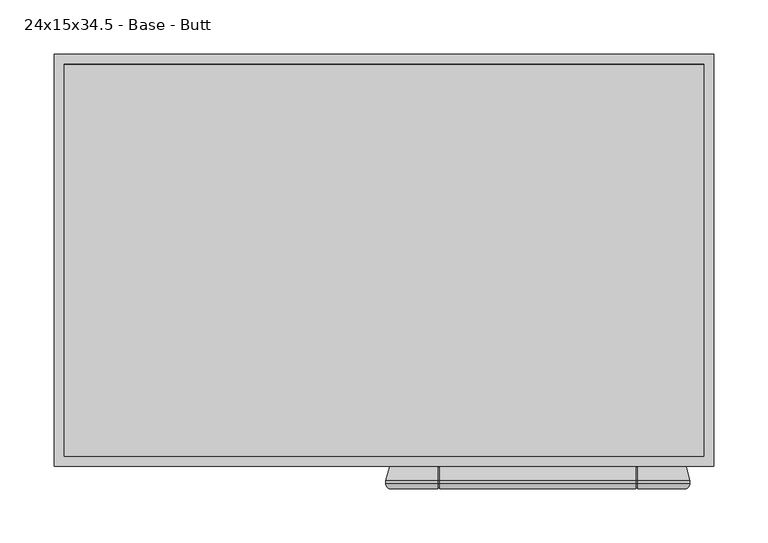
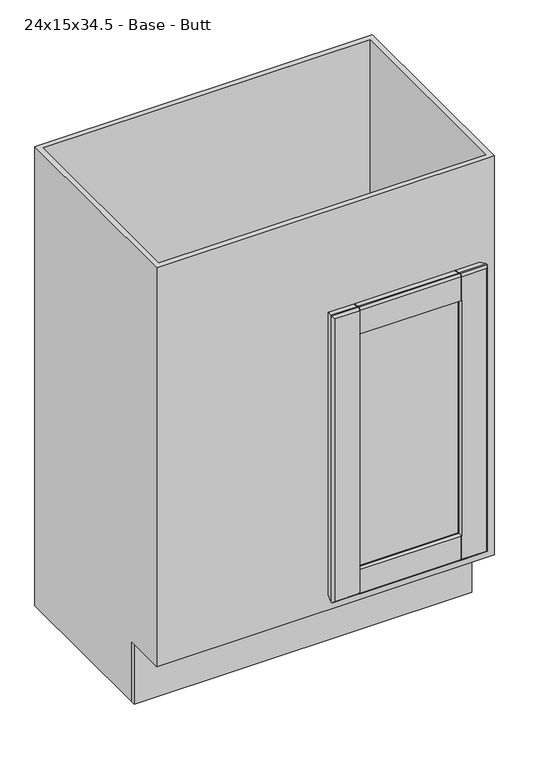
"""IFC4 building model written with IfcOpenShell, lengths in millimetres: furniture geometry, Cabinet-Base-Merillat-Double_Door-Marlin : 24x15x34.5 - Base - Butt."""

from ifc_helpers import new_model, si_unit, frame, origin, origin_with_axes, place, context, project, spatial, polyline, circle_curve, ellipse_curve, outline, extrude, faceted_brep, source, transform, mapped, element, save
from ifc_brep_helpers import plane_surface, cylinder_surface, advanced_brep


def furniture_24x15x34_5_base_butt_ddcd1996(model_context):
    return source(origin(), model_context, "Body", "SolidModel", [
        advanced_brep(
        [(301.3127049, -625.4496, 685.8), (298.2162124, -629.92, 682.7035075), (298.2162124, -629.92, 142.7964925), (301.3127049, -625.4496, 139.7), (301.3127049, -622.681, 139.7), (301.3127049, -622.681, 685.8), (297.8075049, -609.6, 143.2052), (297.8075049, -609.6, 682.2948), (253.1115422, -609.6, 637.5988372), (253.1115422, -609.6, 187.9011628), (252.7414105, -610.39375, 188.2712945), (250.6602514, -614.85681, 190.3524535), (250.6602514, -614.85681, 635.1475465), (252.7414105, -610.39375, 637.2287055), (252.0600209, -617.0969093, 188.952684), (252.0600209, -617.0969093, 636.547316), (266.3877049, -617.347, 174.625), (266.3877049, -617.347, 650.875), (266.3877049, -622.173, 174.625), (266.3877049, -622.173, 650.875), (252.0600209, -622.4230907, 188.952684), (252.0600209, -622.4230907, 636.547316), (250.6602514, -624.66319, 190.3524535), (250.6602514, -624.66319, 635.1475465), (252.7414105, -629.12625, 188.2712945), (253.1086747, -629.9138508, 187.9040302), (253.1115422, -629.92, 637.5988372), (252.7414105, -629.12625, 637.2287055), (253.1086747, -629.92, 142.7964925), (253.1086747, -625.4496, 139.7), (23.4216974, -629.92, 142.7964925), (20.3252049, -625.4496, 139.7), (68.4894236, -625.4496, 139.7), (68.4894236, -629.92, 142.7964925), (251.5211747, -625.4496, 139.7), (251.5211747, -629.92, 142.7964925), (70.0769236, -629.92, 142.7964925), (70.0769236, -625.4496, 139.7), (253.1086747, -622.681, 139.7), (20.3252049, -622.681, 139.7), (68.4894236, -622.681, 139.7), (251.5211747, -622.681, 139.7), (70.0769236, -622.681, 139.7), (253.1086747, -609.6, 143.2052), (23.8304049, -609.6, 143.2052), (68.4894236, -609.6, 143.2052), (251.5211747, -609.6, 143.2052), (70.0769236, -609.6, 143.2052), (70.9776584, -614.85681, 190.3524535), (251.5211747, -610.39375, 188.2712945), (251.5211747, -609.6, 187.9011628), (70.0769236, -609.6, 187.9011628), (70.0769236, -610.39375, 188.2712945), (68.8964994, -610.39375, 188.2712945), (69.577889, -617.0969093, 188.952684), (55.2502049, -617.347, 174.625), (55.2502049, -622.173, 174.625), (69.577889, -622.4230907, 188.952684), (70.9776584, -624.66319, 190.3524535), (68.8964994, -629.12625, 188.2712945), (70.0769236, -629.12625, 188.2712945), (70.0769236, -629.92, 187.9011628), (251.5211747, -629.92, 187.9011628), (251.5211747, -629.12625, 188.2712945), (23.4216974, -629.92, 682.7035075), (20.3252049, -625.4496, 685.8), (20.3252049, -622.681, 685.8), (23.8304049, -609.6, 682.2948), (68.5263677, -609.6, 187.9011628), (68.5263677, -609.6, 637.5988372), (68.8964994, -610.39375, 637.2287055), (70.9776584, -614.85681, 635.1475465), (69.577889, -617.0969093, 636.547316), (55.2502049, -617.347, 650.875), (55.2502049, -622.173, 650.875), (69.577889, -622.4230907, 636.547316), (70.9776584, -624.66319, 635.1475465), (68.8964994, -629.12625, 637.2287055), (68.5263677, -629.92, 637.5988372), (68.5263677, -629.92, 187.9011628), (68.4894236, -629.92, 682.7035075), (68.4894236, -625.4496, 685.8), (253.1086747, -625.4496, 685.8), (253.1086747, -629.92, 682.7035075), (70.0769236, -625.4496, 685.8), (70.0769236, -629.92, 682.7035075), (251.5211747, -629.92, 682.7035075), (251.5211747, -625.4496, 685.8), (68.4894236, -622.681, 685.8), (253.1086747, -622.681, 685.8), (70.0769236, -622.681, 685.8), (251.5211747, -622.681, 685.8), (68.4894236, -609.6, 682.2948), (253.1086747, -609.6, 682.2948), (70.0769236, -609.6, 682.2948), (251.5211747, -609.6, 682.2948), (70.0769236, -609.6, 637.5988372), (251.5211747, -609.6, 637.5988372), (70.0769236, -610.39375, 637.2287055), (251.5211747, -610.39375, 637.2287055), (251.5211747, -629.12625, 637.2287055), (251.5211747, -629.92, 637.5988372), (70.0769236, -629.92, 637.5988372), (70.0769236, -629.12625, 637.2287055), (70.0769236, -610.39375, 681.6857412), (70.0769236, -622.7855037, 685.00625), (70.0769236, -625.4496, 685.00625), (70.0769236, -629.12625, 682.5526052), (68.4894236, -629.12625, 637.2287055), (68.4894236, -629.12625, 682.5526052), (68.4894236, -625.4496, 685.00625), (68.4894236, -622.7855037, 685.00625), (68.4894236, -610.39375, 681.6857412), (68.4894236, -610.39375, 637.2287055), (253.1086747, -610.39375, 637.2287055), (253.1086747, -610.39375, 681.6857412), (253.1086747, -622.7855037, 685.00625), (253.1086747, -625.4496, 685.00625), (253.1086747, -629.12625, 682.5526052), (253.1086747, -629.12625, 637.2287055), (251.5211747, -629.12625, 682.5526052), (251.5211747, -625.4496, 685.00625), (251.5211747, -622.7855037, 685.00625), (251.5211747, -610.39375, 681.6857412), (253.1086747, -629.12625, 188.2712945), (253.1086747, -629.12625, 142.9473948), (253.1086747, -625.4496, 140.49375), (253.1086747, -622.7855037, 140.49375), (253.1086747, -610.39375, 143.8142588), (253.1086747, -610.39375, 188.2712945), (251.5211747, -610.39375, 143.8142588), (251.5211747, -622.7855037, 140.49375), (251.5211747, -625.4496, 140.49375), (251.5211747, -629.12625, 142.9473948), (70.0769236, -629.12625, 142.9473948), (70.0769236, -625.4496, 140.49375), (70.0769236, -622.7855037, 140.49375), (70.0769236, -610.39375, 143.8142588), (68.4894236, -629.12625, 188.2712945), (68.4894236, -610.39375, 188.2712945), (68.4894236, -610.39375, 143.8142588), (68.4894236, -622.7855037, 140.49375), (68.4894236, -625.4496, 140.49375), (68.4894236, -629.12625, 142.9473948)],
        [
            (0, 1, ellipse_curve(frame((296.5375049, -625.4496, 681.0248), z_axis=(0.7071067811865475, 0.0, -0.7071067811865475), x_axis=(0.7071067811865474, 0.0, 0.7071067811865476)), 6.7531526, 4.7752)),
            (1, 2),
            (2, 3, ellipse_curve(frame((296.5375049, -625.4496, 144.4752), z_axis=(0.7071067811865475, 0.0, 0.7071067811865475), x_axis=(-0.7071067811865474, 0.0, 0.7071067811865476)), 6.7531526, 4.7752)),
            (3, 0),
            (3, 4),
            (4, 5),
            (5, 0),
            (4, 6),
            (6, 7),
            (7, 5),
            (8, 9),
            (9, 10),
            (10, 11),
            (11, 12),
            (12, 13),
            (13, 8),
            (11, 14, ellipse_curve(frame((252.0875049, -615.5223492, 188.9252), z_axis=(0.7071067811865475, 0.0, 0.7071067811865475), x_axis=(-0.7071067811865474, 0.0, 0.7071067811865476)), 2.2271035, 1.5748)),
            (14, 15),
            (15, 12, ellipse_curve(frame((252.0875049, -615.5223492, 636.5748), z_axis=(0.7071067811865475, 0.0, -0.7071067811865475), x_axis=(0.7071067811865474, 0.0, 0.7071067811865476)), 2.2271035, 1.5748)),
            (14, 16),
            (16, 17),
            (17, 15),
            (16, 18),
            (18, 19),
            (19, 17),
            (18, 20),
            (20, 21),
            (21, 19),
            (20, 22, ellipse_curve(frame((252.0875049, -623.9976508, 188.9252), z_axis=(0.7071067811865475, 0.0, 0.7071067811865475), x_axis=(-0.7071067811865474, 0.0, 0.7071067811865476)), 2.2271035, 1.5748)),
            (22, 23),
            (23, 21, ellipse_curve(frame((252.0875049, -623.9976508, 636.5748), z_axis=(0.7071067811865475, 0.0, -0.7071067811865475), x_axis=(0.7071067811865474, 0.0, 0.7071067811865476)), 2.2271035, 1.5748)),
            (22, 24),
            (24, 25),
            (25, 26),
            (26, 27),
            (27, 23),
            (2, 28),
            (28, 29, circle_curve(frame((253.1086747, -625.4496, 144.4752), z_axis=(1.0, 0.0, 0.0), x_axis=(0.0, 1.0, 0.0)), 4.7752)),
            (29, 3),
            (30, 31, ellipse_curve(frame((25.1004049, -625.4496, 144.4752), z_axis=(0.7071067811865475, 0.0, -0.7071067811865475), x_axis=(0.7071067811865476, 0.0, 0.7071067811865474)), 6.7531526, 4.7752)),
            (31, 32),
            (32, 33, circle_curve(frame((68.4894236, -625.4496, 144.4752), z_axis=(-1.0, 0.0, 0.0), x_axis=(0.0, 1.0, 0.0)), 4.7752)),
            (33, 30),
            (34, 35, circle_curve(frame((251.5211747, -625.4496, 144.4752), z_axis=(-1.0, 0.0, 0.0), x_axis=(0.0, 1.0, 0.0)), 4.7752)),
            (35, 36),
            (36, 37, circle_curve(frame((70.0769236, -625.4496, 144.4752), z_axis=(1.0, 0.0, 0.0), x_axis=(0.0, 1.0, 0.0)), 4.7752)),
            (37, 34),
            (29, 38),
            (38, 4),
            (31, 39),
            (39, 40),
            (40, 32),
            (41, 34),
            (37, 42),
            (42, 41),
            (38, 43),
            (43, 6),
            (39, 44),
            (44, 45),
            (45, 40),
            (46, 41),
            (42, 47),
            (47, 46),
            (48, 11),
            (10, 49),
            (49, 50),
            (50, 51),
            (51, 52),
            (52, 53),
            (53, 48),
            (48, 54, ellipse_curve(frame((69.5504049, -615.5223492, 188.9252), z_axis=(0.7071067811865475, 0.0, -0.7071067811865475), x_axis=(0.7071067811865476, 0.0, 0.7071067811865474)), 2.2271035, 1.5748)),
            (54, 14),
            (54, 55),
            (55, 16),
            (55, 56),
            (56, 18),
            (56, 57),
            (57, 20),
            (57, 58, ellipse_curve(frame((69.5504049, -623.9976508, 188.9252), z_axis=(0.7071067811865475, 0.0, -0.7071067811865475), x_axis=(0.7071067811865476, 0.0, 0.7071067811865474)), 2.2271035, 1.5748)),
            (58, 22),
            (58, 59),
            (59, 60),
            (60, 61),
            (61, 62),
            (62, 63),
            (63, 24),
            (30, 64),
            (64, 65, ellipse_curve(frame((25.1004049, -625.4496, 681.0248), z_axis=(-0.7071067811865475, 0.0, -0.7071067811865475), x_axis=(0.7071067811865474, 0.0, -0.7071067811865476)), 6.7531526, 4.7752)),
            (65, 31),
            (65, 66),
            (66, 39),
            (66, 67),
            (67, 44),
            (68, 69),
            (69, 70),
            (70, 71),
            (71, 48),
            (53, 68),
            (71, 72, ellipse_curve(frame((69.5504049, -615.5223492, 636.5748), z_axis=(-0.7071067811865475, 0.0, -0.7071067811865475), x_axis=(0.7071067811865474, 0.0, -0.7071067811865476)), 2.2271035, 1.5748)),
            (72, 54),
            (72, 73),
            (73, 55),
            (73, 74),
            (74, 56),
            (74, 75),
            (75, 57),
            (75, 76, ellipse_curve(frame((69.5504049, -623.9976508, 636.5748), z_axis=(-0.7071067811865475, 0.0, -0.7071067811865475), x_axis=(0.7071067811865474, 0.0, -0.7071067811865476)), 2.2271035, 1.5748)),
            (76, 58),
            (76, 77),
            (77, 78),
            (78, 79),
            (79, 59),
            (64, 80),
            (80, 81, circle_curve(frame((68.4894236, -625.4496, 681.0248), z_axis=(-1.0, 0.0, 0.0), x_axis=(0.0, 1.0, 0.0)), 4.7752)),
            (81, 65),
            (0, 82),
            (82, 83, circle_curve(frame((253.1086747, -625.4496, 681.0248), z_axis=(1.0, 0.0, 0.0), x_axis=(0.0, 1.0, 0.0)), 4.7752)),
            (83, 1),
            (84, 85, circle_curve(frame((70.0769236, -625.4496, 681.0248), z_axis=(1.0, 0.0, 0.0), x_axis=(0.0, 1.0, 0.0)), 4.7752)),
            (85, 86),
            (86, 87, circle_curve(frame((251.5211747, -625.4496, 681.0248), z_axis=(-1.0, 0.0, 0.0), x_axis=(0.0, 1.0, 0.0)), 4.7752)),
            (87, 84),
            (81, 88),
            (88, 66),
            (5, 89),
            (89, 82),
            (90, 84),
            (87, 91),
            (91, 90),
            (88, 92),
            (92, 67),
            (7, 93),
            (93, 89),
            (94, 90),
            (91, 95),
            (95, 94),
            (43, 9),
            (8, 93),
            (92, 69),
            (68, 45),
            (96, 94),
            (95, 97),
            (97, 96),
            (50, 46),
            (47, 51),
            (12, 71),
            (70, 98),
            (98, 96),
            (97, 99),
            (99, 13),
            (15, 72),
            (17, 73),
            (19, 74),
            (21, 75),
            (23, 76),
            (27, 100),
            (100, 101),
            (101, 102),
            (102, 103),
            (103, 77),
            (83, 26),
            (25, 28),
            (33, 79),
            (78, 80),
            (85, 102),
            (101, 86),
            (35, 62),
            (61, 36),
            (98, 104),
            (104, 105),
            (105, 106),
            (106, 107, circle_curve(frame((70.0769236, -625.4496, 681.0248), z_axis=(1.0, 0.0, 0.0), x_axis=(0.0, 0.0, 1.0)), 3.98145)),
            (107, 103),
            (78, 108),
            (108, 109),
            (109, 110, circle_curve(frame((68.4894236, -625.4496, 681.0248), z_axis=(-1.0, 0.0, 0.0), x_axis=(0.0, 0.0, 1.0)), 3.98145)),
            (110, 111),
            (111, 112),
            (112, 113),
            (113, 69),
            (77, 108),
            (107, 109),
            (106, 110),
            (105, 111),
            (104, 112),
            (70, 113),
            (8, 114),
            (114, 115),
            (115, 116),
            (116, 117),
            (117, 118, circle_curve(frame((253.1086747, -625.4496, 681.0248), z_axis=(1.0, 0.0, 0.0), x_axis=(0.0, 0.0, 1.0)), 3.98145)),
            (118, 119),
            (119, 26),
            (100, 120),
            (120, 121, circle_curve(frame((251.5211747, -625.4496, 681.0248), z_axis=(-1.0, 0.0, 0.0), x_axis=(0.0, 0.0, 1.0)), 3.98145)),
            (121, 122),
            (122, 123),
            (123, 99),
            (119, 27),
            (118, 120),
            (117, 121),
            (116, 122),
            (115, 123),
            (114, 13),
            (25, 124),
            (124, 125),
            (125, 126, circle_curve(frame((253.1086747, -625.4496, 144.4752), z_axis=(1.0, 0.0, 0.0), x_axis=(0.0, 0.0, 1.0)), 3.98145)),
            (126, 127),
            (127, 128),
            (128, 129),
            (129, 9),
            (49, 130),
            (130, 131),
            (131, 132),
            (132, 133, circle_curve(frame((251.5211747, -625.4496, 144.4752), z_axis=(-1.0, 0.0, 0.0), x_axis=(0.0, 0.0, 1.0)), 3.98145)),
            (133, 63),
            (129, 10),
            (128, 130),
            (127, 131),
            (126, 132),
            (125, 133),
            (124, 24),
            (60, 134),
            (134, 135, circle_curve(frame((70.0769236, -625.4496, 144.4752), z_axis=(1.0, 0.0, 0.0), x_axis=(0.0, 0.0, 1.0)), 3.98145)),
            (135, 136),
            (136, 137),
            (137, 52),
            (138, 79),
            (68, 139),
            (139, 140),
            (140, 141),
            (141, 142),
            (142, 143, circle_curve(frame((68.4894236, -625.4496, 144.4752), z_axis=(-1.0, 0.0, 0.0), x_axis=(0.0, 0.0, 1.0)), 3.98145)),
            (143, 138),
            (138, 59),
            (53, 139),
            (137, 140),
            (136, 141),
            (135, 142),
            (134, 143),
        ],
        [
            cylinder_surface(frame((296.5375049, -625.4496, 685.8), z_axis=(0.0, 0.0, 1.0), x_axis=(0.0, 1.0, 0.0)), 4.7752),
            plane_surface(frame((301.3127049, -625.4496, 685.8), z_axis=(1.0, 0.0, 0.0), x_axis=(0.0, 0.0, -1.0))),
            plane_surface(frame((301.3127049, -622.681, 685.8), z_axis=(0.9659229350723619, 0.25882983502910506, 0.0), x_axis=(0.0, 0.0, -1.0))),
            plane_surface(frame((253.1115422, -609.6, 637.5988372), z_axis=(-0.9063077870366099, 0.4226182617407856, 0.0), x_axis=(0.0, 0.0, -1.0))),
            cylinder_surface(frame((252.0875049, -615.5223492, 685.8), z_axis=(0.0, 0.0, 1.0000000000000002), x_axis=(-0.01745240643729364, -0.9998476951563912, 0.0)), 1.5748),
            plane_surface(frame((252.0600209, -617.0969093, 636.547316), z_axis=(-0.017452406437322144, -0.9998476951563906, 0.0), x_axis=(0.0, 0.0, -1.0))),
            plane_surface(frame((266.3877049, -617.347, 650.875), z_axis=(-1.0, 0.0, 0.0), x_axis=(0.0, 0.0, -1.0))),
            plane_surface(frame((266.3877049, -622.173, 650.875), z_axis=(-0.01745240643727848, 0.9998476951563914, 0.0), x_axis=(0.0, 0.0, -1.0))),
            cylinder_surface(frame((252.0875049, -623.9976508, 685.8), z_axis=(0.0, 0.0, 1.0000000000000002), x_axis=(-0.9063077870367326, -0.42261826174052236, 0.0)), 1.5748),
            plane_surface(frame((250.6602514, -624.66319, 635.1475465), z_axis=(-0.9063077870366333, -0.4226182617407352, 0.0), x_axis=(0.0, 0.0, -1.0))),
            cylinder_surface(frame((301.3127049, -625.4496, 144.4752), z_axis=(1.0, 0.0, 0.0), x_axis=(0.0, 1.0, 0.0)), 4.7752),
            plane_surface(frame((301.3127049, -625.4496, 139.7), z_axis=(0.0, 0.0, -1.0), x_axis=(-1.0, 0.0, 0.0))),
            plane_surface(frame((301.3127049, -622.681, 139.7), z_axis=(0.0, 0.25882983502910506, -0.9659229350723619), x_axis=(-1.0, 0.0, 0.0))),
            plane_surface(frame((253.1115422, -609.6, 187.9011628), z_axis=(0.0, 0.4226182617407856, 0.9063077870366099), x_axis=(-1.0, 0.0, 0.0))),
            cylinder_surface(frame((301.3127049, -615.5223492, 188.9252), z_axis=(1.0000000000000002, 0.0, 0.0), x_axis=(0.0, -0.9998476951563912, 0.01745240643729364)), 1.5748),
            plane_surface(frame((252.0600209, -617.0969093, 188.952684), z_axis=(0.0, -0.9998476951563906, 0.017452406437322144), x_axis=(-1.0, 0.0, 0.0))),
            plane_surface(frame((266.3877049, -617.347, 174.625), z_axis=(0.0, 0.0, 1.0), x_axis=(-1.0, 0.0, 0.0))),
            plane_surface(frame((266.3877049, -622.173, 174.625), z_axis=(0.0, 0.9998476951563914, 0.01745240643727848), x_axis=(-1.0, 0.0, 0.0))),
            cylinder_surface(frame((301.3127049, -623.9976508, 188.9252), z_axis=(1.0000000000000002, 0.0, 0.0), x_axis=(0.0, -0.42261826174052236, 0.9063077870367326)), 1.5748),
            plane_surface(frame((250.6602514, -624.66319, 190.3524535), z_axis=(0.0, -0.4226182617407352, 0.9063077870366333), x_axis=(-1.0, 0.0, 0.0))),
            cylinder_surface(frame((25.1004049, -625.4496, 139.7), z_axis=(0.0, 0.0, -1.0), x_axis=(0.0, 1.0, 0.0)), 4.7752),
            plane_surface(frame((20.3252049, -625.4496, 139.7), z_axis=(-1.0, 0.0, 0.0), x_axis=(0.0, 0.0, 1.0))),
            plane_surface(frame((20.3252049, -622.681, 139.7), z_axis=(-0.9659229350723619, 0.25882983502910506, 0.0), x_axis=(0.0, 0.0, 1.0))),
            plane_surface(frame((68.5263677, -609.6, 187.9011628), z_axis=(0.9063077870366099, 0.4226182617407856, 0.0), x_axis=(0.0, 0.0, 1.0))),
            cylinder_surface(frame((69.5504049, -615.5223492, 139.7), z_axis=(0.0, 0.0, -1.0000000000000002), x_axis=(0.01745240643729364, -0.9998476951563912, 0.0)), 1.5748),
            plane_surface(frame((69.577889, -617.0969093, 188.952684), z_axis=(0.017452406437322144, -0.9998476951563906, 0.0), x_axis=(0.0, 0.0, 1.0))),
            plane_surface(frame((55.2502049, -617.347, 174.625), z_axis=(1.0, 0.0, 0.0), x_axis=(0.0, 0.0, 1.0))),
            plane_surface(frame((55.2502049, -622.173, 174.625), z_axis=(0.01745240643727848, 0.9998476951563914, 0.0), x_axis=(0.0, 0.0, 1.0))),
            cylinder_surface(frame((69.5504049, -623.9976508, 139.7), z_axis=(0.0, 0.0, -1.0000000000000002), x_axis=(0.9063077870367326, -0.42261826174052236, 0.0)), 1.5748),
            plane_surface(frame((70.9776584, -624.66319, 190.3524535), z_axis=(0.9063077870366333, -0.4226182617407352, 0.0), x_axis=(0.0, 0.0, 1.0))),
            cylinder_surface(frame((20.3252049, -625.4496, 681.0248), z_axis=(-1.0, 0.0, 0.0), x_axis=(0.0, 1.0, 0.0)), 4.7752),
            plane_surface(frame((20.3252049, -625.4496, 685.8), z_axis=(0.0, 0.0, 1.0), x_axis=(1.0, 0.0, 0.0))),
            plane_surface(frame((20.3252049, -622.681, 685.8), z_axis=(0.0, 0.25882983502910506, 0.9659229350723619), x_axis=(1.0, 0.0, 0.0))),
            plane_surface(frame((23.8304049, -609.6, 682.2948), z_axis=(0.0, 1.0, 0.0), x_axis=(1.0, 0.0, 0.0))),
            plane_surface(frame((68.5263677, -609.6, 637.5988372), z_axis=(0.0, 0.4226182617407856, -0.9063077870366099), x_axis=(1.0, 0.0, 0.0))),
            cylinder_surface(frame((20.3252049, -615.5223492, 636.5748), z_axis=(-1.0000000000000002, 0.0, 0.0), x_axis=(0.0, -0.9998476951563912, -0.01745240643729364)), 1.5748),
            plane_surface(frame((69.577889, -617.0969093, 636.547316), z_axis=(0.0, -0.9998476951563906, -0.017452406437322144), x_axis=(1.0, 0.0, 0.0))),
            plane_surface(frame((55.2502049, -617.347, 650.875), z_axis=(0.0, 0.0, -1.0), x_axis=(1.0, 0.0, 0.0))),
            plane_surface(frame((55.2502049, -622.173, 650.875), z_axis=(0.0, 0.9998476951563914, -0.01745240643727848), x_axis=(1.0, 0.0, 0.0))),
            cylinder_surface(frame((20.3252049, -623.9976508, 636.5748), z_axis=(-1.0000000000000002, 0.0, 0.0), x_axis=(0.0, -0.42261826174052236, -0.9063077870367326)), 1.5748),
            plane_surface(frame((70.9776584, -624.66319, 635.1475465), z_axis=(0.0, -0.4226182617407352, -0.9063077870366333), x_axis=(1.0, 0.0, 0.0))),
            plane_surface(frame((68.5263677, -629.92, 637.5988372), z_axis=(0.0, -1.0, 0.0), x_axis=(1.0, 0.0, 0.0))),
            plane_surface(frame((70.0769236, -629.92, 637.5988372), z_axis=(-1.0, 0.0, 0.0), x_axis=(0.0, 0.906307787036771, -0.4226182617404399))),
            plane_surface(frame((68.4894236, -629.92, 637.5988372), z_axis=(1.0, 0.0, 0.0), x_axis=(0.0, -0.906307787036771, 0.4226182617404399))),
            plane_surface(frame((70.0769236, -629.92, 637.5988372), z_axis=(0.0, 0.4226182617404399, 0.906307787036771), x_axis=(-1.0, 0.0, 0.0))),
            plane_surface(frame((70.0769236, -629.12625, 637.2287055), z_axis=(0.0, -1.0, 0.0), x_axis=(-1.0, 0.0, 0.0))),
            cylinder_surface(frame((68.4894236, -625.4496, 681.0248), z_axis=(-1.0, 0.0, 0.0), x_axis=(0.0, 0.0, 1.0)), 3.98145),
            plane_surface(frame((70.0769236, -625.4496, 685.00625), z_axis=(0.0, 0.0, 1.0), x_axis=(-1.0, 0.0, 0.0))),
            plane_surface(frame((70.0769236, -622.7855037, 685.00625), z_axis=(0.0, 0.25882983502913415, 0.9659229350723542), x_axis=(-1.0, 0.0, 0.0))),
            plane_surface(frame((70.0769236, -610.39375, 681.6857412), z_axis=(0.0, 1.0, 0.0), x_axis=(-1.0, 0.0, 0.0))),
            plane_surface(frame((70.0769236, -610.39375, 637.2287055), z_axis=(0.0, -0.4226182617405111, 0.9063077870367379), x_axis=(-1.0, 0.0, 0.0))),
            plane_surface(frame((253.1086747, -629.92, 637.5988372), z_axis=(-1.0, 0.0, 0.0), x_axis=(0.0, 0.9063077870367783, -0.42261826174042444))),
            plane_surface(frame((251.5211747, -629.92, 637.5988372), z_axis=(1.0, 0.0, 0.0), x_axis=(0.0, -0.9063077870367783, 0.42261826174042444))),
            plane_surface(frame((253.1086747, -629.92, 637.5988372), z_axis=(0.0, 0.42261826174042444, 0.9063077870367783), x_axis=(-1.0, 0.0, 0.0))),
            plane_surface(frame((253.1086747, -629.12625, 637.2287055), z_axis=(0.0, -1.0, 0.0), x_axis=(-1.0, 0.0, 0.0))),
            cylinder_surface(frame((251.5211747, -625.4496, 681.0248), z_axis=(-1.0, 0.0, 0.0), x_axis=(0.0, 0.0, 1.0)), 3.98145),
            plane_surface(frame((253.1086747, -625.4496, 685.00625), z_axis=(0.0, 0.0, 1.0), x_axis=(-1.0, 0.0, 0.0))),
            plane_surface(frame((253.1086747, -622.7855037, 685.00625), z_axis=(0.0, 0.25882983502911566, 0.965922935072359), x_axis=(-1.0, 0.0, 0.0))),
            plane_surface(frame((253.1086747, -610.39375, 681.6857412), z_axis=(0.0, 1.0, 0.0), x_axis=(-1.0, 0.0, 0.0))),
            plane_surface(frame((253.1086747, -610.39375, 637.2287055), z_axis=(0.0, -0.42261826174056427, 0.9063077870367131), x_axis=(-1.0, 0.0, 0.0))),
            plane_surface(frame((253.1086747, -625.4496, 149.2504), z_axis=(-1.0, 0.0, 0.0), x_axis=(0.0, -1.0, 0.0))),
            plane_surface(frame((251.5211747, -625.4496, 149.2504), z_axis=(1.0, 0.0, 0.0), x_axis=(0.0, 1.0, 0.0))),
            plane_surface(frame((253.1086747, -609.6, 187.9011628), z_axis=(0.0, -0.42261826173999295, -0.9063077870369795), x_axis=(-1.0, 0.0, 0.0))),
            plane_surface(frame((253.1086747, -610.39375, 188.2712945), z_axis=(0.0, 1.0, 0.0), x_axis=(-1.0, 0.0, 0.0))),
            plane_surface(frame((253.1086747, -610.39375, 143.8142588), z_axis=(0.0, 0.2588298350290845, -0.9659229350723675), x_axis=(-1.0, 0.0, 0.0))),
            plane_surface(frame((253.1086747, -622.7855037, 140.49375), z_axis=(0.0, 0.0, -1.0), x_axis=(-1.0, 0.0, 0.0))),
            cylinder_surface(frame((251.5211747, -625.4496, 144.4752), z_axis=(-1.0, 0.0, 0.0), x_axis=(0.0, 0.0, 1.0)), 3.98145),
            plane_surface(frame((253.1086747, -629.12625, 142.9473948), z_axis=(0.0, -1.0, 0.0), x_axis=(-1.0, 0.0, 0.0))),
            plane_surface(frame((253.1086747, -629.12625, 188.2712945), z_axis=(0.0, 0.4226182617407698, -0.9063077870366172), x_axis=(-1.0, 0.0, 0.0))),
            plane_surface(frame((70.0769236, -629.12625, 188.2712945), z_axis=(-1.0, 0.0, 0.0), x_axis=(0.0, -0.906307787036583, -0.42261826174084305))),
            plane_surface(frame((68.4894236, -629.12625, 188.2712945), z_axis=(1.0, 0.0, 0.0), x_axis=(0.0, 0.906307787036583, 0.42261826174084305))),
            plane_surface(frame((70.0769236, -629.12625, 188.2712945), z_axis=(0.0, 0.42261826174084305, -0.906307787036583), x_axis=(-1.0, 0.0, 0.0))),
            plane_surface(frame((70.0769236, -609.6, 187.9011628), z_axis=(0.0, -0.42261826174073325, -0.9063077870366342), x_axis=(-1.0, 0.0, 0.0))),
            plane_surface(frame((70.0769236, -610.39375, 188.2712945), z_axis=(0.0, 1.0, 0.0), x_axis=(-1.0, 0.0, 0.0))),
            plane_surface(frame((70.0769236, -610.39375, 143.8142588), z_axis=(0.0, 0.2588298350290967, -0.9659229350723642), x_axis=(-1.0, 0.0, 0.0))),
            plane_surface(frame((70.0769236, -622.7855037, 140.49375), z_axis=(0.0, 0.0, -1.0), x_axis=(-1.0, 0.0, 0.0))),
            cylinder_surface(frame((68.4894236, -625.4496, 144.4752), z_axis=(-1.0, 0.0, 0.0), x_axis=(0.0, 0.0, 1.0)), 3.98145),
            plane_surface(frame((70.0769236, -629.12625, 142.9473948), z_axis=(0.0, -1.0, 0.0), x_axis=(-1.0, 0.0, 0.0))),
        ],
        [
            (0, [[1, 2, 3, 4]]),
            (1, [[-4, 5, 6, 7]]),
            (2, [[-6, 8, 9, 10]]),
            (3, [[11, 12, 13, 14, 15, 16]]),
            (4, [[-14, 17, 18, 19]]),
            (5, [[-18, 20, 21, 22]]),
            (6, [[-21, 23, 24, 25]]),
            (7, [[-24, 26, 27, 28]]),
            (8, [[-27, 29, 30, 31]]),
            (9, [[-30, 32, 33, 34, 35, 36]]),
            (10, [[-3, 37, 38, 39]]),
            (10, [[40, 41, 42, 43]]),
            (10, [[44, 45, 46, 47]]),
            (11, [[-5, -39, 48, 49]]),
            (11, [[50, 51, 52, -41]]),
            (11, [[53, -47, 54, 55]]),
            (12, [[-8, -49, 56, 57]]),
            (12, [[58, 59, 60, -51]]),
            (12, [[61, -55, 62, 63]]),
            (13, [[64, -13, 65, 66, 67, 68, 69, 70]]),
            (14, [[-17, -64, 71, 72]]),
            (15, [[-20, -72, 73, 74]]),
            (16, [[-23, -74, 75, 76]]),
            (17, [[-26, -76, 77, 78]]),
            (18, [[-29, -78, 79, 80]]),
            (19, [[-80, 81, 82, 83, 84, 85, 86, -32]]),
            (20, [[-40, 87, 88, 89]]),
            (21, [[-50, -89, 90, 91]]),
            (22, [[-58, -91, 92, 93]]),
            (23, [[94, 95, 96, 97, -70, 98]]),
            (24, [[-71, -97, 99, 100]]),
            (25, [[-73, -100, 101, 102]]),
            (26, [[-75, -102, 103, 104]]),
            (27, [[-77, -104, 105, 106]]),
            (28, [[-79, -106, 107, 108]]),
            (29, [[-108, 109, 110, 111, 112, -81]]),
            (30, [[-88, 113, 114, 115]]),
            (30, [[-1, 116, 117, 118]]),
            (30, [[119, 120, 121, 122]]),
            (31, [[-90, -115, 123, 124]]),
            (31, [[-7, 125, 126, -116]]),
            (31, [[127, -122, 128, 129]]),
            (32, [[-92, -124, 130, 131]]),
            (32, [[-10, 132, 133, -125]]),
            (32, [[134, -129, 135, 136]]),
            (33, [[-9, -57, 137, -11, 138, -132]]),
            (33, [[-93, -131, 139, -94, 140, -59]]),
            (33, [[141, -136, 142, 143]]),
            (33, [[144, -63, 145, -67]]),
            (34, [[146, -96, 147, 148, -143, 149, 150, -15]]),
            (35, [[-19, 151, -99, -146]]),
            (36, [[-22, 152, -101, -151]]),
            (37, [[-25, 153, -103, -152]]),
            (38, [[-28, 154, -105, -153]]),
            (39, [[-31, 155, -107, -154]]),
            (40, [[-155, -36, 156, 157, 158, 159, 160, -109]]),
            (41, [[-2, -118, 161, -34, 162, -37]]),
            (41, [[-87, -43, 163, -111, 164, -113]]),
            (41, [[165, -158, 166, -120]]),
            (41, [[167, -84, 168, -45]]),
            (42, [[169, 170, 171, 172, 173, -159, -165, -119, -127, -134, -141, -148]]),
            (43, [[174, 175, 176, 177, 178, 179, 180, -139, -130, -123, -114, -164]]),
            (44, [[-174, -110, 181]]),
            (45, [[-173, 182, -175, -181, -160]]),
            (46, [[-172, 183, -176, -182]]),
            (47, [[-171, 184, -177, -183]]),
            (48, [[-170, 185, -178, -184]]),
            (49, [[-169, -147, 186, -179, -185]]),
            (50, [[-180, -186, -95]]),
            (51, [[187, 188, 189, 190, 191, 192, 193, -161, -117, -126, -133, -138]]),
            (52, [[194, 195, 196, 197, 198, -149, -142, -135, -128, -121, -166, -157]]),
            (53, [[-193, 199, -35]]),
            (54, [[-192, 200, -194, -156, -199]]),
            (55, [[-191, 201, -195, -200]]),
            (56, [[-190, 202, -196, -201]]),
            (57, [[-189, 203, -197, -202]]),
            (58, [[-188, 204, -150, -198, -203]]),
            (59, [[-187, -16, -204]]),
            (60, [[205, 206, 207, 208, 209, 210, 211, -137, -56, -48, -38, -162]]),
            (61, [[212, 213, 214, 215, 216, -85, -167, -44, -53, -61, -144, -66]]),
            (62, [[-211, 217, -12]]),
            (63, [[-210, 218, -212, -65, -217]]),
            (64, [[-209, 219, -213, -218]]),
            (65, [[-208, 220, -214, -219]]),
            (66, [[-207, 221, -215, -220]]),
            (67, [[-206, 222, -86, -216, -221]]),
            (68, [[-205, -33, -222]]),
            (69, [[223, 224, 225, 226, 227, -68, -145, -62, -54, -46, -168, -83]]),
            (70, [[228, -163, -42, -52, -60, -140, 229, 230, 231, 232, 233, 234]]),
            (71, [[-228, 235, -112]]),
            (72, [[-229, -98, 236]]),
            (73, [[-227, 237, -230, -236, -69]]),
            (74, [[-226, 238, -231, -237]]),
            (75, [[-225, 239, -232, -238]]),
            (76, [[-224, 240, -233, -239]]),
            (77, [[-223, -82, -235, -234, -240]]),
        ],
    ),
        extrude(outline(polyline([(55.2502049, -622.173), (55.2502049, -617.347), (266.3877049, -617.347), (266.3877049, -622.173), (55.2502049, -622.173)])), frame((0.0, 0.0, 174.625), z_axis=(0.0, 0.0, 1.0), x_axis=(1.0, 0.0, 0.0)), (0.0, 0.0, 1.0), 476.25),
        faceted_brep([(323.5377049, -228.6, 0.0), (323.5377049, -529.43125, 0.0), (314.0127049, -529.43125, 0.0), (314.0127049, -238.125, 0.0), (-276.5372951, -238.125, 0.0), (-276.5372951, -529.43125, 0.0), (-286.0622951, -529.43125, 0.0), (-286.0622951, -228.6, 0.0), (-286.0622951, -228.6, 876.3), (323.5377049, -228.6, 876.3), (-286.0622951, -529.43125, 114.3), (-286.0622951, -609.6, 114.3), (-286.0622951, -609.6, 876.3), (323.5377049, -609.6, 876.3), (323.5377049, -609.6, 114.3), (323.5377049, -529.43125, 114.3), (314.0127049, -529.43125, 114.3), (314.0127049, -238.125, 114.3), (314.0127049, -600.075, 876.3), (314.0127049, -238.125, 876.3), (314.0127049, -238.125, 123.825), (314.0127049, -600.075, 123.825), (-276.5372951, -238.125, 114.3), (-276.5372951, -529.43125, 114.3), (-276.5372951, -238.125, 876.3), (-276.5372951, -600.075, 876.3), (-276.5372951, -600.075, 123.825), (-276.5372951, -238.125, 123.825)], [[[0, 1, 2, 3, 4, 5, 6, 7]], [[0, 7, 8, 9]], [[7, 6, 10, 11, 12, 8]], [[1, 0, 9, 13, 14, 15]], [[3, 2, 16, 17]], [[18, 19, 20, 21]], [[5, 4, 22, 23]], [[24, 25, 26, 27]], [[4, 3, 17, 22]], [[19, 24, 27, 20]], [[9, 8, 12, 13], [19, 18, 25, 24]], [[14, 11, 10, 23, 22, 17, 16, 15]], [[13, 12, 11, 14]], [[25, 18, 21, 26]], [[6, 5, 23, 10]], [[2, 1, 15, 16]], [[21, 20, 27, 26]]]),
        extrude(outline(polyline([(323.5377049, -529.43125), (323.5377049, -538.95625), (-286.0622951, -538.95625), (-286.0622951, -529.43125), (323.5377049, -529.43125)])), origin_with_axes(), (0.0, 0.0, 1.0), 114.3),
    ])


if __name__ == "__main__":
    model = new_model("IFC4")
    model_context = context("Model", 3, world=origin())
    ifc_project = project(units=[si_unit("LENGTHUNIT", "METRE", prefix="MILLI")], contexts=[model_context])
    site = spatial("IfcSite", under=ifc_project)
    building = spatial("IfcBuilding", under=site)
    placement = place(None, origin())
    furniture_24x15x34_5_base_butt_shape = furniture_24x15x34_5_base_butt_ddcd1996(model_context)
    element("IfcFurniture", 1, ObjectType="Cabinet-Base-Merillat-Double_Door-Marlin : 24x15x34.5 - Base - Butt", at=placement, inside=building, context=model_context, shape_type="MappedRepresentation", body=[
        mapped(furniture_24x15x34_5_base_butt_shape, transform((0.0, 0.0, 0.0), x_axis=(1.0, 0.0, 0.0), y_axis=(0.0, 1.0, 0.0), z_axis=(0.0, 0.0, 1.0))),
    ])
    save(model, "model.ifc")

# Revit data of these elements
# Type "Cabinet-Base-Merillat-Double_Door-Marlin : 24x15x34.5 - Base - Butt"
#   URL = "http://www.merillat.com"
#   Toe Kick Note = "Toe Kick Covering is not included. To be purchased Separately."
#   Product Line = "Express"
#   Product Page URL = "http://www.merillat.com//our-products/rooms/kitchen"
#   Product Group = "Base Cabinet"
#   Product Documentation Link = "http://merillatbusiness.com/customer-resources/product-line-resources/merillat-classic/"
#   Model = "B24B"
#   Manufacturer = "Merillat"
#   Finish = "Wood"
#   Description = "Base Butt Door"
#   Construction Type = "Deep Sink Base"
#   Cabinet Construction Note = "BUTT doors without a center frame stile, For tray or shelf option,  replace HDS with the option code of your choice,  When depth is reduced  to 12\" or 15\" drawer becomes false front"
#   Assembly Code = "C1030410"
#   Toe Kick Height = 0' - 4 1/2"
#   Toe Kick Depth = 0' - 2 25/32"
#   Top and Bottom Spacing = 0' - 1"
#   Side Spacing = 0' - 0 7/8"
#   Cabinet Shell = 0' - 0 3/8"
#   Door Spacing = 0' - 0 1/8"
#   Depth = 1' - 3"
#   Height = 2' - 10 1/2"
#   Width = 2' - 0"
#   Cabinet Drawer Width = 1' - 10 1/4"
#   Cabinet Drawer Height = 0' - 5 1/2"
#   Cabinet Drawer 2 Drawer Width = 0' - 11 1/16"
#   Cabinet Door Width = 0' - 11 1/16"
#   Cabinet Door Height = 1' - 9 1/2"
#   COBie.Type = no
#   Two Drawer = no
#   Elevation Swing Line = yes
#   Partial Overlay = yes
#   One Drawer = yes
#   Full Overlay = no
#   Butt Option = yes
#   Toe Kick Material = Wood - Merillat - Raw Particle Board
#   Door Drawer Material = Wood - Merillat - Pecan(1)
#   Cabinet Material = Wood - Merillat - Pecan(1)
#   Cabinet Drawer Style 2 Drawer = element 819256
#   Cabinet Drawer Style = element 819255
#   Cabinet Door Style = element 819254
# Element 1 (IfcFurniture, "Cabinet-Base-Merillat-Double_Door-Marlin : 24x15x34.5 - Base - Butt")
#   Materials on its faces: "Wood - Merillat - Pecan(1)", "Wood - Merillat - Raw Particle Board"
# Materials
#   "Wood - Merillat - Raw Particle Board": class "Plastic", colour RGB 80 80 80, transparency 0, Description = "Plastic Laminate - Navy", Cost = 0
#   "Wood - Merillat - Pecan(1)": class "Wood", colour RGB 108 67 43, transparency 0, Cost = 0
